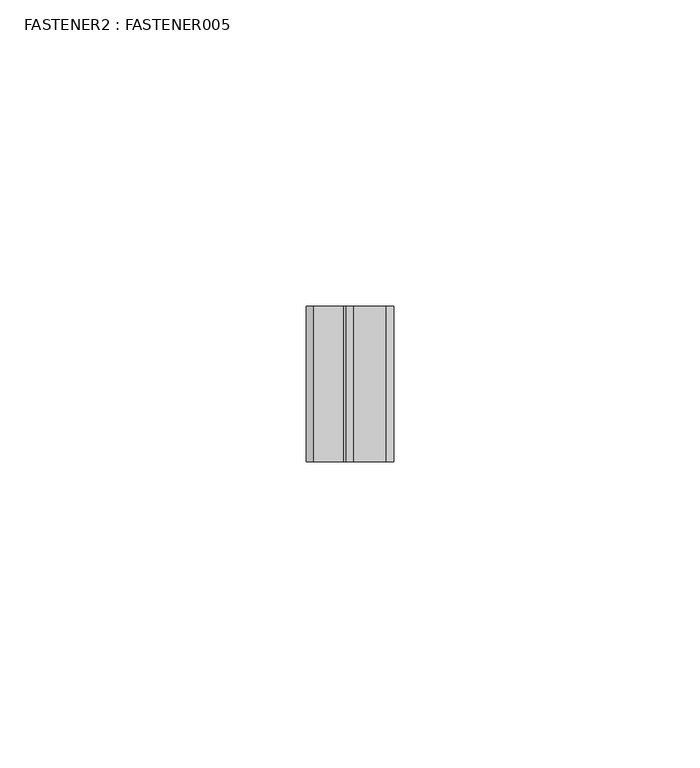
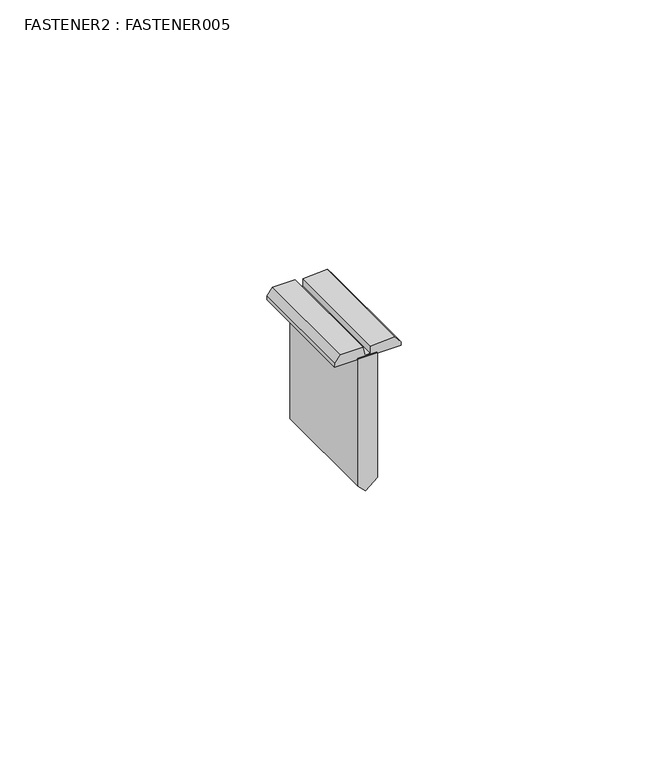
"""IFC4 building model written with IfcOpenShell, lengths in millimetres: proxy geometry, FASTENER2 : FASTENER005."""

from ifc_helpers import new_model, si_unit, frame, origin, place, context, project, spatial, polyline, outline, extrude, source, transform, mapped, element, save


def fastener2_fastener005_4a0cef2c(model_context):
    return source(origin(), model_context, "Body", "SweptSolid", [
        extrude(outline(polyline([(42579.6987049, 5977.3107075), (42550.7399648, 5977.3107075), (42549.1244121, 5978.9677221), (42551.3049701, 5981.517626), (42579.6987049, 5981.517626), (42579.6987049, 5977.3107075)])), frame((0.0, -1078.2906574, 0.0), z_axis=(0.0, 1.0, 0.0), x_axis=(0.0, 0.0, 1.0)), (0.0, 0.0, 1.0), 25.4),
        extrude(outline(polyline([(42579.6987049, 5986.5634932), (42580.508527, 5986.5634932), (42582.1023984, 5985.3247911), (42581.7061629, 5980.0391089), (42580.1167322, 5980.0391089), (42580.1167322, 5978.792004), (42582.1288635, 5978.3957685), (42582.1288635, 5973.5166866), (42580.5349921, 5972.2779845), (42579.6987049, 5972.2671879), (42579.6987049, 5986.5634932)])), frame((0.0, -1078.2906574, 0.0), z_axis=(0.0, 1.0, 0.0), x_axis=(0.0, 0.0, 1.0)), (0.0, 0.0, 1.0), 25.4),
    ])


if __name__ == "__main__":
    model = new_model("IFC4")
    model_context = context("Model", 3, world=origin())
    ifc_project = project(units=[si_unit("LENGTHUNIT", "METRE", prefix="MILLI")], contexts=[model_context])
    site = spatial("IfcSite", under=ifc_project)
    building = spatial("IfcBuilding", under=site)
    placement = place(None, origin())
    fastener2_fastener005_shape = fastener2_fastener005_4a0cef2c(model_context)
    element("IfcBuildingElementProxy", 1, Name="FASTENER2 : FASTENER005", ObjectType="FASTENER2 : FASTENER005", at=placement, inside=building, context=model_context, shape_type="MappedRepresentation", body=[
        mapped(fastener2_fastener005_shape, transform((0.0, 0.0, 0.0), x_axis=(1.0, 0.0, 0.0), y_axis=(0.0, 1.0, 0.0), z_axis=(0.0, 0.0, 1.0))),
    ])
    save(model, "model.ifc")

# Revit data of these elements
# Type "FASTENER2 : FASTENER005"
#   NameOverride = "FASTENER005"
# Element 1 (IfcBuildingElementProxy, "FASTENER2 : FASTENER005")
#   Materials on its faces: "ENGINEERED PANCAKE HEAD FASTENER (NOT BY AEP-SPAN) @ 12\" O.C."
# Materials
#   "ENGINEERED PANCAKE HEAD FASTENER (NOT BY AEP-SPAN) @ 12\" O.C.": class "Unassigned", colour RGB 255 255 255, transparency 0
